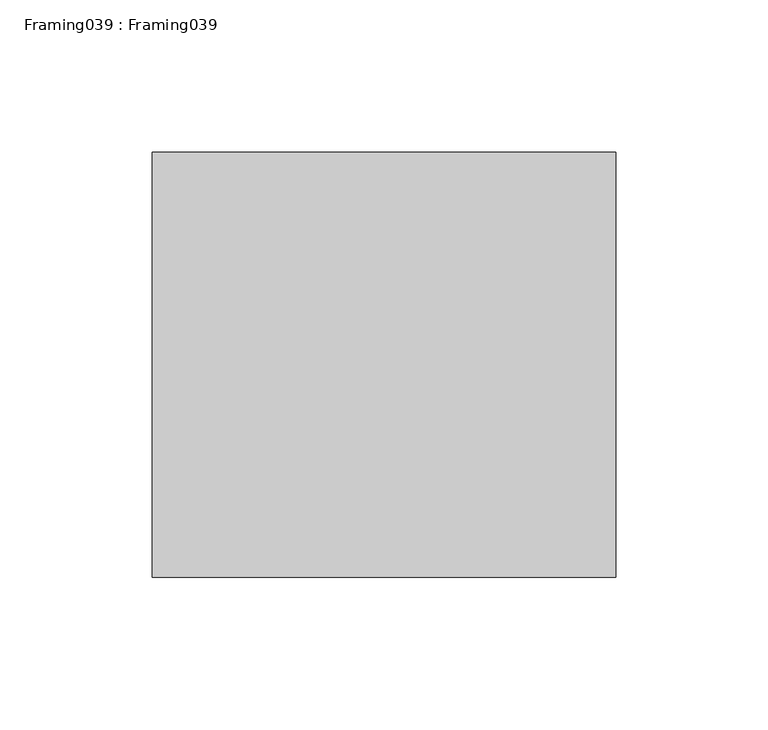
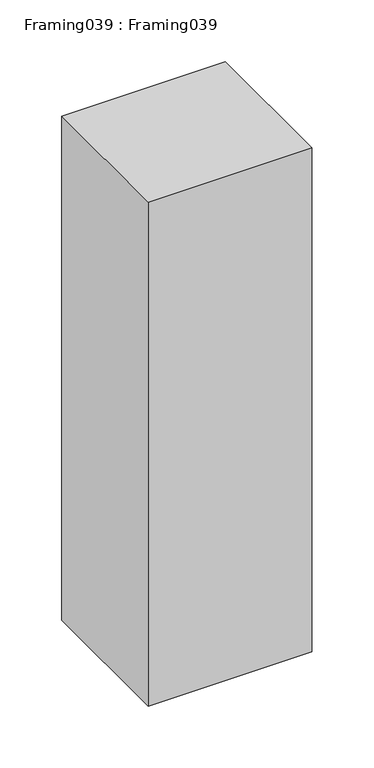
"""IFC4 building model written with IfcOpenShell, lengths in millimetres: proxy geometry, Framing039 : Framing039."""

from ifc_helpers import new_model, si_unit, frame, origin, place, context, project, spatial, polyline, outline, extrude, source, transform, mapped, element, save


def framing039_framing039_e4e9f5ad(model_context):
    return source(origin(), model_context, "Body", "SweptSolid", [
        extrude(outline(polyline([(13535.4175781, -4497.8424805), (13535.4175781, -4637.5424805), (13383.0175781, -4637.5424805), (13383.0175781, -4497.8424805), (13535.4175781, -4497.8424805)])), frame((0.0, 0.0, 39158.796875), z_axis=(0.0, 0.0, 1.0), x_axis=(1.0, 0.0, 0.0)), (0.0, 0.0, 1.0), 496.699125),
    ])


if __name__ == "__main__":
    model = new_model("IFC4")
    model_context = context("Model", 3, world=origin())
    ifc_project = project(units=[si_unit("LENGTHUNIT", "METRE", prefix="MILLI")], contexts=[model_context])
    site = spatial("IfcSite", under=ifc_project)
    building = spatial("IfcBuilding", under=site)
    placement = place(None, origin())
    framing039_framing039_shape = framing039_framing039_e4e9f5ad(model_context)
    element("IfcBuildingElementProxy", 1, Name="Framing039 : Framing039", ObjectType="Framing039 : Framing039", at=placement, inside=building, context=model_context, shape_type="MappedRepresentation", body=[
        mapped(framing039_framing039_shape, transform((0.0, 0.0, 0.0), x_axis=(1.0, 0.0, 0.0), y_axis=(0.0, 1.0, 0.0), z_axis=(0.0, 0.0, 1.0))),
    ])
    save(model, "model.ifc")

# Revit data of these elements
# Type "Framing039 : Framing039"
#   NameOverride = "Framing039"
# Element 1 (IfcBuildingElementProxy, "Framing039 : Framing039")
#   Materials on its faces: "WOOD FRAMING (SEE STRUCT DWGS)"
# Materials
#   "WOOD FRAMING (SEE STRUCT DWGS)": class "Unassigned", colour RGB 224 188 168, transparency 0, Cost = 0
